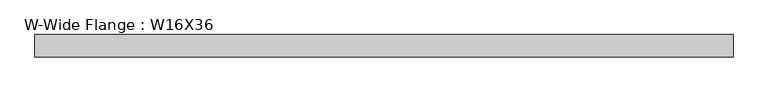
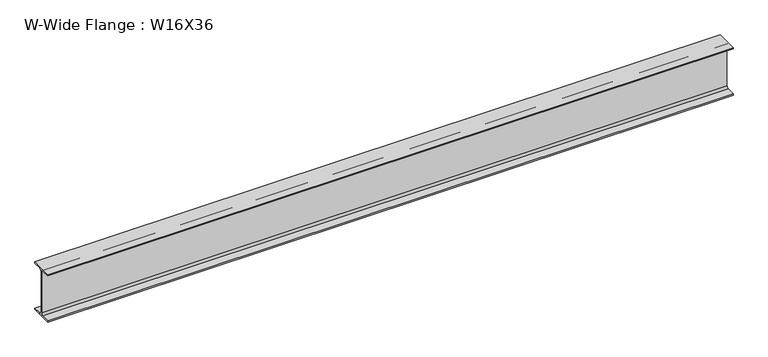
"""IFC4 building model written with IfcOpenShell, lengths in millimetres: beam geometry, W-Wide Flange : W16X36."""

from ifc_helpers import new_model, si_unit, point, frame, frame_2d, origin, place, context, project, spatial, polyline, circle_curve, trimmed, segment, composite_curve, outline, extrude, source, transform, mapped, element, save


def w_wide_flange_w16x36_23a21d2c(model_context):
    return source(origin(), model_context, "Body", "SweptSolid", [
        extrude(outline(composite_curve([segment(polyline([(88.773, -191.008), (88.773, -201.93), (-88.773, -201.93), (-88.773, -191.008), (-21.3995, -191.008)]), True, "CONTINUOUS"), segment(trimmed(circle_curve(frame_2d((-21.3995, -173.355)), 17.653), [point((-21.3995, -191.008))], [point((-3.7465, -173.355))], True, "CARTESIAN"), True, "CONTINUOUS"), segment(polyline([(-3.7465, -173.355), (-3.7465, 173.355)]), True, "CONTINUOUS"), segment(trimmed(circle_curve(frame_2d((-21.3995, 173.355)), 17.653), [point((-3.7465, 173.355))], [point((-21.3995, 191.008))], True, "CARTESIAN"), True, "CONTINUOUS"), segment(polyline([(-21.3995, 191.008), (-88.773, 191.008), (-88.773, 201.93), (88.773, 201.93), (88.773, 191.008), (21.3995, 191.008)]), True, "CONTINUOUS"), segment(trimmed(circle_curve(frame_2d((21.3995, 173.355)), 17.653), [point((21.3995, 191.008))], [point((3.7465, 173.355))], True, "CARTESIAN"), True, "CONTINUOUS"), segment(polyline([(3.7465, 173.355), (3.7465, -173.355)]), True, "CONTINUOUS"), segment(trimmed(circle_curve(frame_2d((21.3995, -173.355)), 17.653), [point((3.7465, -173.355))], [point((21.3995, -191.008))], True, "CARTESIAN"), True, "CONTINUOUS"), segment(polyline([(21.3995, -191.008), (88.773, -191.008)]), True, "CONTINUOUS")], self_intersect=False)), frame((-2755.9, 0.0, 0.0), z_axis=(1.0, 0.0, 0.0), x_axis=(0.0, 1.0, 0.0)), (0.0, 0.0, 1.0), 5511.8),
    ])


if __name__ == "__main__":
    model = new_model("IFC4")
    model_context = context("Model", 3, world=origin())
    ifc_project = project(units=[si_unit("LENGTHUNIT", "METRE", prefix="MILLI")], contexts=[model_context])
    site = spatial("IfcSite", under=ifc_project)
    building = spatial("IfcBuilding", under=site)
    placement = place(None, origin())
    w_wide_flange_w16x36_shape = w_wide_flange_w16x36_23a21d2c(model_context)
    element("IfcBeam", 1, ObjectType="W-Wide Flange : W16X36", at=placement, inside=building, context=model_context, shape_type="MappedRepresentation", body=[
        mapped(w_wide_flange_w16x36_shape, transform((0.0, 0.0, 0.0), x_axis=(1.0, 0.0, 0.0), y_axis=(0.0, 1.0, 0.0), z_axis=(0.0, 0.0, 1.0))),
    ])
    save(model, "model.ifc")

# Revit data of these elements
# Type "W-Wide Flange : W16X36"
#   Assembly Code = "B10"
#   W = 36
#   Length [instance default] = 5' - 0"
#   bf = 0' - 6.99"
#   d = 1' - 3.9"
#   k = 0' - 1 1/8"
#   k2 = 0' - 0.695"
#   tf = 0' - 0.43"
#   tw = 0' - 0.295"
#   A = 0.0736111 SF
#   Structural Material [instance default] = Steel ASTM A992
# Element 1 (IfcBeam, "W-Wide Flange : W16X36")
#   Materials on its faces: "Steel ASTM A992"
# Materials
#   "Steel ASTM A992": class "Metal", colour RGB 199 199 199, transparency 0, Description = "Structural steel 50ksi", Cost = 0
